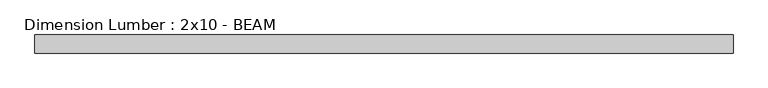
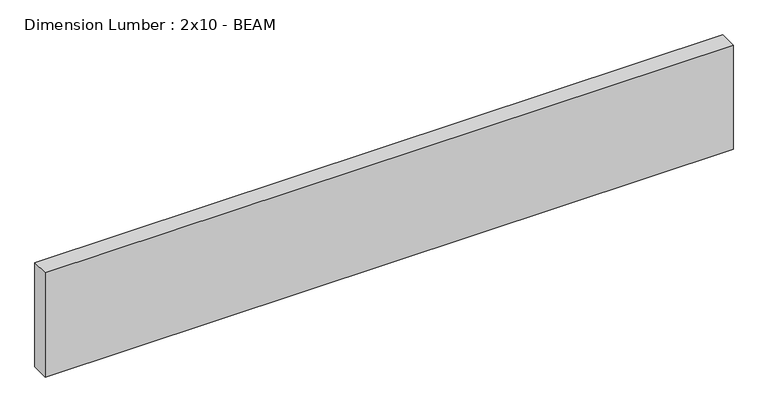
"""IFC4 building model written with IfcOpenShell, lengths in millimetres: beam geometry, Dimension Lumber : 2x10 - BEAM."""

from ifc_helpers import new_model, si_unit, frame, origin, place, context, project, spatial, polyline, outline, extrude, source, transform, mapped, element, save


def dimension_lumber_2x10_beam_6cc76e73(model_context):
    return source(origin(), model_context, "Body", "SweptSolid", [
        extrude(outline(polyline([(782.7119141, 19.05), (782.7119141, -19.05), (-685.8744141, -19.05), (-685.8744141, 19.05), (782.7119141, 19.05)])), frame((0.0, 0.0, -117.475), z_axis=(0.0, 0.0, 1.0), x_axis=(1.0, 0.0, 0.0)), (0.0, 0.0, 1.0), 234.95),
    ])


if __name__ == "__main__":
    model = new_model("IFC4")
    model_context = context("Model", 3, world=origin())
    ifc_project = project(units=[si_unit("LENGTHUNIT", "METRE", prefix="MILLI")], contexts=[model_context])
    site = spatial("IfcSite", under=ifc_project)
    building = spatial("IfcBuilding", under=site)
    placement = place(None, origin())
    dimension_lumber_2x10_beam_shape = dimension_lumber_2x10_beam_6cc76e73(model_context)
    element("IfcBeam", 1, ObjectType="Dimension Lumber : 2x10 - BEAM", at=placement, inside=building, context=model_context, shape_type="MappedRepresentation", body=[
        mapped(dimension_lumber_2x10_beam_shape, transform((0.0, 0.0, 0.0), x_axis=(1.0, 0.0, 0.0), y_axis=(0.0, 1.0, 0.0), z_axis=(0.0, 0.0, 1.0))),
    ])
    save(model, "model.ifc")

# Revit data of these elements
# Type "Dimension Lumber : 2x10 - BEAM"
#   Assembly Code = "B10"
#   A = 0.0755556 SF
#   Length [instance default] = 5' - 0"
#   b = 0' - 1 1/2"
#   d = 0' - 9 1/4"
#   Structural Material = (3) SISTERED 2X10s AT BEAM
# Element 1 (IfcBeam, "Dimension Lumber : 2x10 - BEAM")
#   Materials on its faces: "(3) SISTERED 2X10s AT BEAM"
# Materials
#   "(3) SISTERED 2X10s AT BEAM": class "Wood", colour RGB 234 198 147, transparency 0, Description = "Pinus Echinata", Cost = 0
